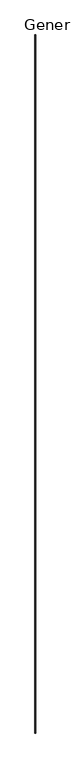
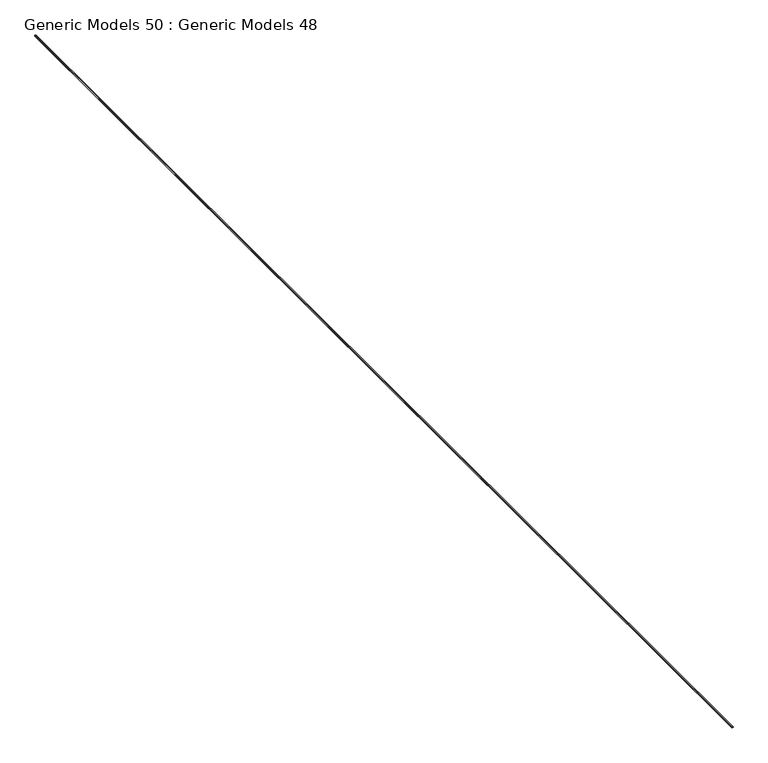
"""IFC4 building model written with IfcOpenShell, lengths in millimetres: proxy geometry, Generic Models 50 : Generic Models 48."""

from ifc_helpers import new_model, si_unit, point, frame, origin, place, context, project, spatial, polyline, circle_curve, ellipse_curve, trimmed, source, transform, mapped, element, save
from ifc_brep_helpers import plane_surface, cylinder_surface, revolved_surface, extruded_surface, advanced_brep


def generic_models_50_generic_models_48_8317c953(model_context):
    return source(origin(), model_context, "Body", "AdvancedBrep", [
        advanced_brep(
        [(32118.8568886, 29574.9917286, 269371.8011404), (32118.8568886, 29574.9917286, 269365.4511404), (32122.0318886, 29574.9917286, 269365.4511404), (32122.983648, 29574.9917286, 269366.721799), (32122.983648, 29574.9917286, 269370.5304819), (32122.0318886, 29574.9917286, 269371.8011404), (32118.8568886, 40781.6231612, 269371.8011404), (32122.0318886, 40781.6231612, 269371.8011404), (32122.983648, 40781.6231612, 269370.5304819), (32122.983648, 40781.6231612, 269366.721799), (32122.0318886, 40781.6231612, 269365.4511404), (32118.8568886, 40781.6231612, 269365.4511404)],
        [
            (0, 1, circle_curve(frame((32115.9421481, 29574.9917286, 269368.6261404), z_axis=(0.0, 1.0, 0.0), x_axis=(0.0, 0.0, 1.0)), 4.3100275)),
            (1, 2),
            (2, 3, circle_curve(frame((32119.1171481, 29574.9917286, 269368.6261404), z_axis=(0.0, -1.0, 0.0), x_axis=(0.0, 0.0, 1.0)), 4.3100275)),
            (3, 4, ellipse_curve(frame((32126.7943886, 29574.9917286, 269368.6261404), z_axis=(0.0, -1.0, 0.0), x_axis=(-1.0, 0.0, 0.0)), 4.7625, 3.175)),
            (4, 5, circle_curve(frame((32119.1171481, 29574.9917286, 269368.6261404), z_axis=(0.0, -1.0, 0.0), x_axis=(0.0, 0.0, 1.0)), 4.3100275)),
            (5, 0),
            (6, 7),
            (7, 8, circle_curve(frame((32119.1171481, 40781.6231612, 269368.6261404), z_axis=(0.0, 1.0, 0.0), x_axis=(0.0, 0.0, 1.0)), 4.3100275)),
            (8, 9, ellipse_curve(frame((32126.7943886, 40781.6231612, 269368.6261404), z_axis=(0.0, 1.0, 0.0), x_axis=(-1.0, 0.0, 0.0)), 4.7625, 3.175)),
            (9, 10, circle_curve(frame((32119.1171481, 40781.6231612, 269368.6261404), z_axis=(0.0, 1.0, 0.0), x_axis=(0.0, 0.0, 1.0)), 4.3100275)),
            (10, 11),
            (11, 6, circle_curve(frame((32115.9421481, 40781.6231612, 269368.6261404), z_axis=(0.0, -1.0, 0.0), x_axis=(0.0, 0.0, 1.0)), 4.3100275)),
            (5, 7),
            (6, 0),
            (4, 8),
            (3, 9),
            (2, 10),
            (1, 11),
        ],
        [
            plane_surface(frame((32118.8568886, 29574.9917286, 269365.4511404), z_axis=(0.0, -1.0, 0.0), x_axis=(1.0, 0.0, 0.0))),
            plane_surface(frame((32118.8568886, 40781.6231612, 269365.4511404), z_axis=(0.0, 1.0, 0.0), x_axis=(1.0, 0.0, 0.0))),
            plane_surface(frame((32122.0318886, 29574.9917286, 269371.8011404), z_axis=(0.0, 0.0, 1.0), x_axis=(0.0, 1.0, 0.0))),
            cylinder_surface(frame((32119.1171481, 29574.9917286, 269368.6261404), z_axis=(0.0, -1.0, 0.0), x_axis=(0.0, 0.0, 1.0)), 4.3100275),
            extruded_surface(trimmed(ellipse_curve(frame((32126.7943886, 40781.6231612, 269368.6261404), z_axis=(0.0, -1.0, 0.0), x_axis=(-1.0, 0.0, 0.0)), 4.7625, 3.175), [point((32122.983648, 40781.6231612, 269366.721799))], [point((32122.983648, 40781.6231612, 269370.5304819))], True, "CARTESIAN"), (0.0, -11206.631432599996, 0.0), 11206.631432599996),
            plane_surface(frame((32118.8568886, 29574.9917286, 269365.4511404), z_axis=(0.0, 0.0, -1.0), x_axis=(0.0, 1.0, 0.0))),
            revolved_surface(polyline([(32115.9421481, 40781.6231612, 269372.9361679), (32115.9421481, 29574.9917286, 269372.9361679)]), (32115.9421481, 29574.9917286, 269368.6261404), (0.0, 1.0, 0.0)),
        ],
        [
            (0, [[1, 2, 3, 4, 5, 6]]),
            (1, [[7, 8, 9, 10, 11, 12]]),
            (2, [[-6, 13, -7, 14]]),
            (3, [[-5, 15, -8, -13]]),
            (4, [[-4, 16, -9, -15]]),
            (3, [[-3, 17, -10, -16]]),
            (5, [[-2, 18, -11, -17]]),
            (6, [[-1, -14, -12, -18]]),
        ],
    ),
    ])


if __name__ == "__main__":
    model = new_model("IFC4")
    model_context = context("Model", 3, world=origin())
    ifc_project = project(units=[si_unit("LENGTHUNIT", "METRE", prefix="MILLI")], contexts=[model_context])
    site = spatial("IfcSite", under=ifc_project)
    building = spatial("IfcBuilding", under=site)
    placement = place(None, origin())
    generic_models_50_generic_models_48_shape = generic_models_50_generic_models_48_8317c953(model_context)
    element("IfcBuildingElementProxy", 1, Name="Generic Models 50 : Generic Models 48", ObjectType="Generic Models 50 : Generic Models 48", at=placement, inside=building, context=model_context, shape_type="MappedRepresentation", body=[
        mapped(generic_models_50_generic_models_48_shape, transform((0.0, 0.0, 0.0), x_axis=(1.0, 0.0, 0.0), y_axis=(0.0, 1.0, 0.0), z_axis=(0.0, 0.0, 1.0))),
    ])
    save(model, "model.ifc")

# Revit data of these elements
# Element 1 (IfcBuildingElementProxy, "Generic Models 50 : Generic Models 48")
#   Materials on its faces: "SEALANT (& BACKER ROD IF NECESSARY)"
# Materials
#   "SEALANT (& BACKER ROD IF NECESSARY)": class "Generic", colour RGB 176 213 108, transparency 0, Cost = 0
